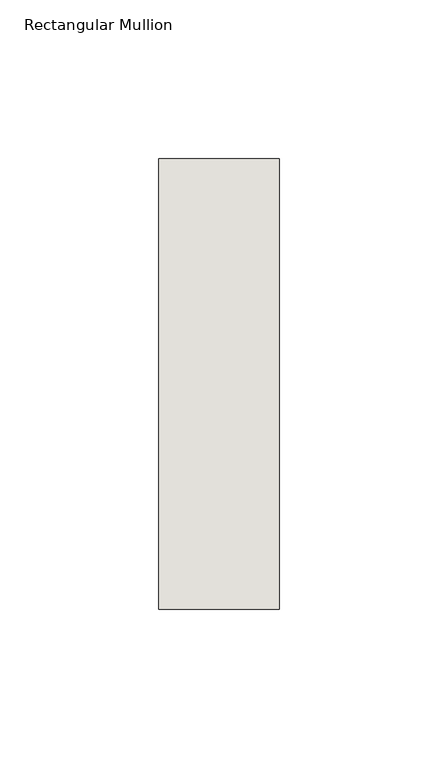
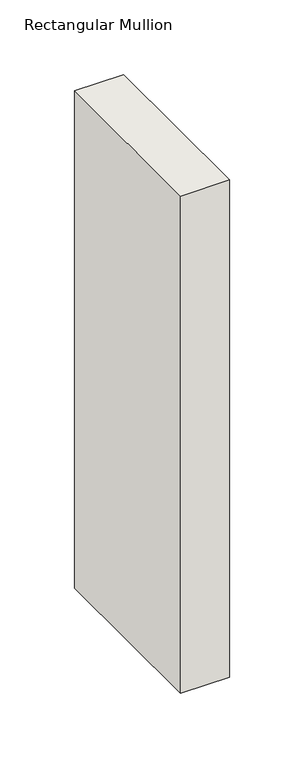
"""IFC4 building model written with IfcOpenShell, lengths in millimetres: wall geometry, Rectangular Mullion : NLRS_21_CWM_hsb-regel 38x142_gen_rsf."""

from ifc_helpers import new_model, si_unit, frame, origin, place, context, project, spatial, polyline, outline, extrude, source, transform, mapped, element, save


def rectangular_mullion_fd8aedfe(model_context):
    return source(origin(), model_context, "Body", "SweptSolid", [
        extrude(outline(polyline([(-38.0, -71.0), (-38.0, 71.0), (0.0, 71.0), (0.0, -71.0), (-38.0, -71.0)])), frame((0.0, 0.0, -407.0), z_axis=(0.0, 0.0, 1.0), x_axis=(1.0, 0.0, 0.0)), (0.0, 0.0, 1.0), 407.0),
    ])


if __name__ == "__main__":
    model = new_model("IFC4")
    model_context = context("Model", 3, world=origin())
    ifc_project = project(units=[si_unit("LENGTHUNIT", "METRE", prefix="MILLI")], contexts=[model_context])
    site = spatial("IfcSite", under=ifc_project)
    building = spatial("IfcBuilding", under=site)
    placement = place(None, origin())
    rectangular_mullion_shape = rectangular_mullion_fd8aedfe(model_context)
    element("IfcWall", 1, ObjectType="Rectangular Mullion : NLRS_21_CWM_hsb-regel 38x142_gen_rsf", at=placement, inside=building, context=model_context, shape_type="MappedRepresentation", body=[
        mapped(rectangular_mullion_shape, transform((0.0, 0.0, 0.0), x_axis=(1.0, 0.0, 0.0), y_axis=(0.0, 1.0, 0.0), z_axis=(0.0, 0.0, 1.0))),
    ])
    save(model, "model.ifc")

# Revit data of these elements
# Type "Rectangular Mullion : NLRS_21_CWM_hsb-regel 38x142_gen_rsf"
#   Type IfcGUID = "07M7mRoiH1CR8m_RSKIwpF"
#   Assembly Code = "21.10"
#   IfcExportAs = "IfcWall"
#   built-in parameter 1007322 = 0.465879 (stored number, unit not read)
#   built-in parameter 1007321 = 0.062336 (stored number, unit not read)
#   built-in parameter 1007320 = 0.062336 (stored number, unit not read)
# Element 1 (IfcWall, "Rectangular Mullion : NLRS_21_CWM_hsb-regel 38x142_gen_rsf")
#   Materials on its faces: "NLRS_i2_hout naaldhout vuren_gen_rsf"
# Materials
#   "NLRS_i2_hout naaldhout vuren_gen_rsf": class "I - Hout", colour RGB 234 199 147, transparency 0, Keynote = "i2", Manufacturer = "Revit Standards Foundation", URL = "www.revitstandards.org", Description = "hout vuren", Cost = 0
